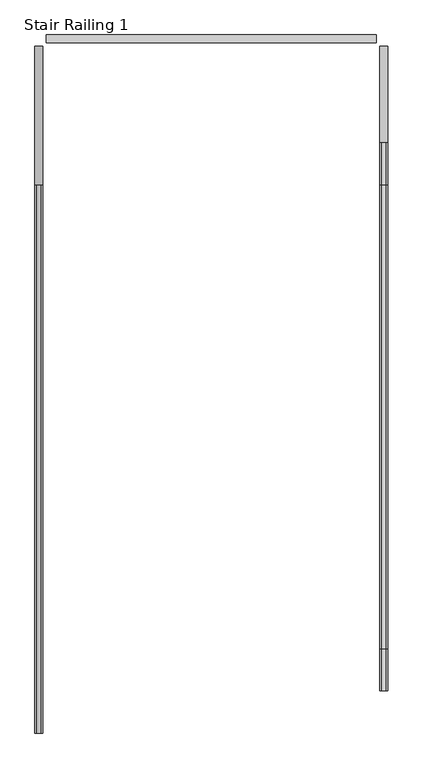
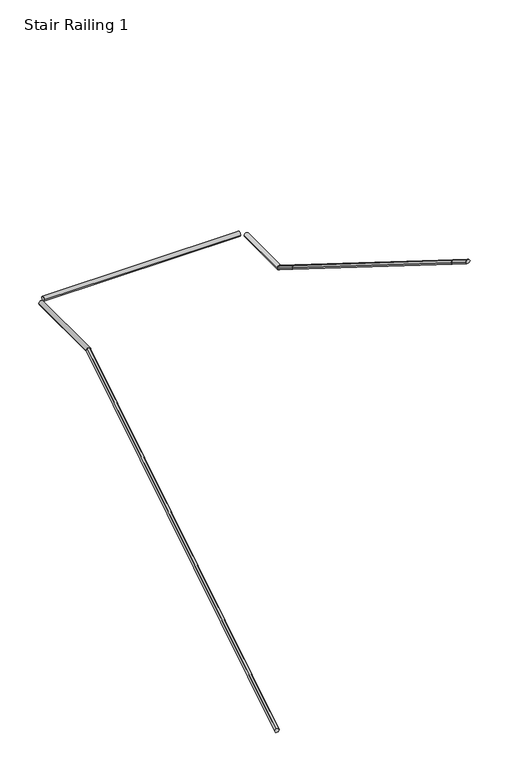
"""IFC4 building model written with IfcOpenShell, lengths in millimetres: railing geometry, Stair Railing 1."""

import ifcopenshell
import ifcopenshell.guid

model = None  # the IFC model being written
_history = None  # IfcOwnerHistory: only IFC2X3 demands one
_inside = {}  # id of a spatial element -> (the spatial element, [elements in it])
_under = {}  # id of a project, library or spatial element -> (it, [spatial elements below it])
_declared = {}  # id of a project -> (the project, [libraries it declares])
_typed = {}  # id of a type object -> (the type object, [elements of that type])
_made_of = {}  # id of a material, layer set ... -> (it, [elements and type objects made of it])


def new_model(schema):
    """Start an empty IFC model of exactly this schema.

    Asked for "IFC4X3", IfcOpenShell would pick the latest addendum, in which some entities
    have other attributes; the version numbers below select the first issue.
    IFC2X3 requires an IfcOwnerHistory on every rooted entity: one is made here for all.
    """
    global model, _history
    if schema == "IFC4X3":
        model = ifcopenshell.file(schema_version=(4, 3, 0, 0))
    else:
        model = ifcopenshell.file(schema=schema)
    _inside.clear()
    _under.clear()
    _declared.clear()
    _typed.clear()
    _made_of.clear()
    _history = None
    if model.schema == "IFC2X3":
        org = make("IfcOrganization", Name="unknown")
        user = make(
            "IfcPersonAndOrganization",
            ThePerson=make("IfcPerson", FamilyName="unknown"),
            TheOrganization=org,
        )
        app = make(
            "IfcApplication",
            ApplicationDeveloper=org,
            Version="unknown",
            ApplicationFullName="unknown",
            ApplicationIdentifier="unknown",
        )
        _history = make(
            "IfcOwnerHistory",
            OwningUser=user,
            OwningApplication=app,
            ChangeAction="ADDED",
            CreationDate=0,
        )
    return model


def make(cls, **values):
    """One entity of the class cls with the attributes given. An attribute that is None is left unset."""
    return model.create_entity(
        cls, **{name: value for name, value in values.items() if value is not None}
    )


def rooted(cls, **values):
    """An entity with a GlobalId (a new one), such as an element, a storey or a relation."""
    return make(cls, GlobalId=ifcopenshell.guid.new(), OwnerHistory=_history, **values)


def si_unit(unit_type, name, prefix=None):
    """IfcSIUnit, for example si_unit("LENGTHUNIT", "METRE", prefix="MILLI")."""
    return make("IfcSIUnit", UnitType=unit_type, Prefix=prefix, Name=name)


def assignment(units):
    """IfcUnitAssignment: the units of a project."""
    return None if units is None else make("IfcUnitAssignment", Units=units)


def point(xyz):
    """IfcCartesianPoint."""
    return None if xyz is None else make("IfcCartesianPoint", Coordinates=xyz)


def direction(xyz):
    """IfcDirection."""
    return None if xyz is None else make("IfcDirection", DirectionRatios=xyz)


def frame(location, z_axis=None, x_axis=None):
    """IfcAxis2Placement3D, a coordinate frame: its origin and axes. An axis left out is left unset."""
    return make(
        "IfcAxis2Placement3D",
        Location=point(location),
        Axis=direction(z_axis),
        RefDirection=direction(x_axis),
    )


def origin():
    """The frame at (0, 0, 0) with its axes left unset."""
    return frame((0.0, 0.0, 0.0))


def place(relative_to, where):
    """IfcLocalPlacement: puts the frame where relative to a parent placement (None: the world)."""
    return make(
        "IfcLocalPlacement", PlacementRelTo=relative_to, RelativePlacement=where
    )


def context(
    kind, dimensions, precision=None, world=None, true_north=None, identifier=None
):
    """IfcGeometricRepresentationContext, for example the 3D "Model" context."""
    return make(
        "IfcGeometricRepresentationContext",
        ContextIdentifier=identifier,
        ContextType=kind,
        CoordinateSpaceDimension=dimensions,
        Precision=precision,
        WorldCoordinateSystem=world,
        TrueNorth=true_north,
    )


def project(units=None, contexts=None):
    """IfcProject with its units and contexts."""
    return rooted(
        "IfcProject",
        Name="project",
        RepresentationContexts=contexts,
        UnitsInContext=assignment(units),
    )


def spatial(cls, under=None, at=None, **own):
    """A site, building, storey or space (cls), placed at a placement, below another one or the project."""
    s = rooted(cls, ObjectPlacement=at, **own)
    if under is not None:
        _under.setdefault(under.id(), (under, []))[1].append(s)
    return s


def circle_curve(where, radius):
    """IfcCircle in the frame where."""
    return make("IfcCircle", Position=where, Radius=radius)


def faces_of(points, faces, orient=None, outer=None):
    """IfcFace entities. A face is a list of loops; a loop is a list of indices into points, from 0.

    orient and outer hold one flag for each loop. By default every Orientation is true, the
    first loop of a face is its IfcFaceOuterBound and the others are IfcFaceBound.
    """
    made = []
    for i, loops in enumerate(faces):
        bounds = []
        for j, loop in enumerate(loops):
            is_outer = j == 0 if outer is None else outer[i][j]
            bounds.append(
                make(
                    "IfcFaceOuterBound" if is_outer else "IfcFaceBound",
                    Bound=make("IfcPolyLoop", Polygon=[points[k] for k in loop]),
                    Orientation=True if orient is None else orient[i][j],
                )
            )
        made.append(make("IfcFace", Bounds=bounds))
    return made


def faceted_brep(points, faces, orient=None, outer=None, voids=None):
    """IfcFacetedBrep: a solid bounded by flat faces; with voids (closed shells), ...WithVoids."""
    shared = [point(p) for p in points]
    hull = make("IfcClosedShell", CfsFaces=faces_of(shared, faces, orient, outer))
    if voids is None:
        return make("IfcFacetedBrep", Outer=hull)
    return make(
        "IfcFacetedBrepWithVoids",
        Outer=hull,
        Voids=[
            make(cls, CfsFaces=faces_of(shared, fs, o, b)) for cls, fs, o, b in voids
        ],
    )


def shape(context_of_items, identifier, shape_type, items):
    """IfcShapeRepresentation: the items that make up one representation, for example the "Body"."""
    return make(
        "IfcShapeRepresentation",
        ContextOfItems=context_of_items,
        RepresentationIdentifier=identifier,
        RepresentationType=shape_type,
        Items=items,
    )


def source(mapping_origin, context_of_items, identifier, shape_type, items):
    """IfcRepresentationMap: a shape defined once, which mapped items show again and again."""
    return make(
        "IfcRepresentationMap",
        MappingOrigin=mapping_origin,
        MappedRepresentation=shape(context_of_items, identifier, shape_type, items),
    )


def transform(
    local_origin,
    x_axis=None,
    y_axis=None,
    z_axis=None,
    scale=None,
    scale2=None,
    scale3=None,
    uniform=True,
):
    """IfcCartesianTransformationOperator3D, or its non-uniform kind. x_axis, y_axis, z_axis: its Axis1, 2, 3."""
    if uniform:
        return make(
            "IfcCartesianTransformationOperator3D",
            Axis1=direction(x_axis),
            Axis2=direction(y_axis),
            LocalOrigin=point(local_origin),
            Scale=scale,
            Axis3=direction(z_axis),
        )
    return make(
        "IfcCartesianTransformationOperator3DnonUniform",
        Axis1=direction(x_axis),
        Axis2=direction(y_axis),
        LocalOrigin=point(local_origin),
        Scale=scale,
        Axis3=direction(z_axis),
        Scale2=scale2,
        Scale3=scale3,
    )


def mapped(mapping_source, mapping_target):
    """IfcMappedItem: shows the shape of a source again, moved by a transform."""
    return make(
        "IfcMappedItem", MappingSource=mapping_source, MappingTarget=mapping_target
    )


def made_of(thing, what):
    """Note that an element or type object is made of a material, layer set ...; save() writes the relation."""
    if what is not None:
        _made_of.setdefault(what.id(), (what, []))[1].append(thing)
    return thing


def element(
    cls,
    number,
    at=None,
    inside=None,
    cuts=None,
    type_object=None,
    material=None,
    context=None,
    identifier="Body",
    shape_type=None,
    held_by="IfcProductDefinitionShape",
    body=None,
    shapes=None,
    **own,
):
    """One element of the class cls, such as IfcWall. Its Tag is "e" and its number.

    at: its placement. inside: the storey or other place that contains it. cuts: it is an
    opening in that element (IfcRelVoidsElement). A single representation is given by context,
    identifier, shape_type and body (its items); several are given by shapes. held_by: the class
    of the entity that holds the representations. save() writes the other relations.
    """
    e = rooted(cls, Tag="e%d" % number, ObjectPlacement=at, **own)
    if body is not None:
        shapes = [shape(context, identifier, shape_type, body)]
    if shapes is not None:
        e.Representation = make(held_by, Representations=shapes)
    if inside is not None:
        _inside.setdefault(inside.id(), (inside, []))[1].append(e)
    if cuts is not None:
        rooted(
            "IfcRelVoidsElement", RelatingBuildingElement=cuts, RelatedOpeningElement=e
        )
    if type_object is not None:
        _typed.setdefault(type_object.id(), (type_object, []))[1].append(e)
    return made_of(e, material)


def aggregate(whole, parts):
    """IfcRelAggregates: a whole, such as a stair, and the parts it consists of."""
    return rooted("IfcRelAggregates", RelatingObject=whole, RelatedObjects=parts)


def save(model, path):
    """Write the relations noted so far, then the file.

    IfcRelAggregates (storeys below a building ...), IfcRelContainedInSpatialStructure (elements
    in a storey), IfcRelDefinesByType, IfcRelAssociatesMaterial and IfcRelDeclares: one each for
    every whole, place, type object, material and project.
    """
    for whole, parts in _under.values():
        aggregate(whole, parts)
    for where, things in _inside.values():
        rooted(
            "IfcRelContainedInSpatialStructure",
            RelatedElements=things,
            RelatingStructure=where,
        )
    for kind, things in _typed.values():
        rooted("IfcRelDefinesByType", RelatedObjects=things, RelatingType=kind)
    for what, things in _made_of.values():
        rooted("IfcRelAssociatesMaterial", RelatedObjects=things, RelatingMaterial=what)
    for by, libraries in _declared.values():
        rooted("IfcRelDeclares", RelatingContext=by, RelatedDefinitions=libraries)
    model.write(path)


def plane_surface(at):
    """IfcPlane: the flat surface through the origin of the frame at, square to its z axis."""
    return make("IfcPlane", Position=at)


def cylinder_surface(at, radius):
    """IfcCylindricalSurface: all points at the distance radius from the z axis of the frame at."""
    return make("IfcCylindricalSurface", Position=at, Radius=radius)


def advanced_brep(points, edges, surfaces, faces):
    """IfcAdvancedBrep: a solid bounded by faces that lie on surfaces and meet in shared edges.

    An edge is (start, end): straight between two places in points (the first is 0);
    or (start, end, curve); or (start, end, curve, False) where it runs against its curve.
    A face is (place in surfaces, loops), or (place, loops, False) where it looks against
    its surface's normal. A loop lists edges by number (the first is 1), with a minus sign
    where the edge is run from its end to its start. The first loop is the outer one.
    """
    corners = [point(p) for p in points]
    vertices = [make("IfcVertexPoint", VertexGeometry=c) for c in corners]
    made = []
    for start, end, *more in edges:
        made.append(
            make(
                "IfcEdgeCurve",
                EdgeStart=vertices[start],
                EdgeEnd=vertices[end],
                EdgeGeometry=more[0] if more else make("IfcPolyline", Points=[corners[start], corners[end]]),
                SameSense=more[1] if len(more) > 1 else True,
            )
        )
    hull = []
    for where, loops, *sense in faces:
        bounds = []
        for j, loop in enumerate(loops):
            ring = [make("IfcOrientedEdge", EdgeElement=made[abs(k) - 1], Orientation=k > 0) for k in loop]
            bounds.append(
                make(
                    "IfcFaceOuterBound" if j == 0 else "IfcFaceBound",
                    Bound=make("IfcEdgeLoop", EdgeList=ring),
                    Orientation=True,
                )
            )
        hull.append(make("IfcAdvancedFace", Bounds=bounds, FaceSurface=surfaces[where], SameSense=sense[0] if sense else True))
    return make("IfcAdvancedBrep", Outer=make("IfcClosedShell", CfsFaces=hull))


def stair_railing_1_2cf15c4a(model_context):
    return source(origin(), model_context, "Body", "SolidModel", [
        faceted_brep([(-2482.1134126, 56357.2066802, 13752.6888889), (-2469.4134126, 56357.2066802, 13774.6859341), (-2444.0134126, 56357.2066802, 13774.6859341), (-2431.3134126, 56357.2066802, 13752.6888889), (-2444.0134126, 56357.2066802, 13730.6918436), (-2469.4134126, 56357.2066802, 13730.6918436), (-2482.1134126, 52725.0066802, 11477.9777778), (-2469.4134126, 52725.0066802, 11455.9807325), (-2444.0134126, 52725.0066802, 11455.9807325), (-2431.3134126, 52725.0066802, 11477.9777778), (-2444.0134126, 52725.0066802, 11499.974823), (-2469.4134126, 52725.0066802, 11499.974823)], [[[0, 1, 2, 3, 4, 5]], [[6, 7, 8, 9, 10, 11]], [[1, 0, 6, 11]], [[2, 1, 11, 10]], [[3, 2, 10, 9]], [[4, 3, 9, 8]], [[5, 4, 8, 7]], [[0, 5, 7, 6]]]),
        advanced_brep(
        [(-2482.1134126, 57271.6066802, 13752.6888889), (-2431.3134126, 57271.6066802, 13752.6888889), (-2482.1134126, 56357.2066802, 13752.6888889), (-2431.3134126, 56357.2066802, 13752.6888889)],
        [
            (0, 1, circle_curve(frame((-2456.7134126, 57271.6066802, 13752.6888889), z_axis=(0.0, 1.0, 0.0), x_axis=(-0.9999999999999999, 0.0, 0.0)), 25.4)),
            (1, 0, circle_curve(frame((-2456.7134126, 57271.6066802, 13752.6888889), z_axis=(0.0, 1.0, 0.0), x_axis=(-0.9999999999999999, 0.0, 0.0)), 25.4)),
            (2, 3, circle_curve(frame((-2456.7134126, 56357.2066802, 13752.6888889), z_axis=(0.0, -1.0, 0.0), x_axis=(-0.9999999999999999, 0.0, 0.0)), 25.4)),
            (3, 2, circle_curve(frame((-2456.7134126, 56357.2066802, 13752.6888889), z_axis=(0.0, -1.0, 0.0), x_axis=(-0.9999999999999999, 0.0, 0.0)), 25.4)),
            (0, 2),
            (3, 1),
        ],
        [
            plane_surface(frame((-2482.1134126, 57271.6066802, 13727.2888889), z_axis=(0.0, 1.0, 0.0), x_axis=(0.0, 0.0, 1.0))),
            plane_surface(frame((-2482.1134126, 56357.2066802, 13727.2888889), z_axis=(0.0, -1.0, 0.0), x_axis=(0.0, 0.0, -1.0))),
            cylinder_surface(frame((-2456.7134126, 56357.2066802, 13752.6888889), z_axis=(0.0, 0.9999999999999999, 0.0), x_axis=(-0.9999999999999999, 0.0, 0.0)), 25.4),
        ],
        [
            (0, [[1, 2]]),
            (1, [[3, 4]]),
            (2, [[-1, 5, -4, 6]]),
            (2, [[-2, -6, -3, -5]]),
        ],
    ),
        advanced_brep(
        [(-222.5891104, 57347.8066802, 13752.6888889), (-222.5891104, 57297.0066802, 13752.6888889), (-2405.9134126, 57347.8066802, 13752.6888889), (-2405.9134126, 57297.0066802, 13752.6888889)],
        [
            (0, 1, circle_curve(frame((-222.5891104, 57322.4066802, 13752.6888889), z_axis=(1.0, 0.0, 0.0), x_axis=(0.0, 1.0, 0.0)), 25.4)),
            (1, 0, circle_curve(frame((-222.5891104, 57322.4066802, 13752.6888889), z_axis=(1.0, 0.0, 0.0), x_axis=(0.0, 1.0, 0.0)), 25.4)),
            (2, 3, circle_curve(frame((-2405.9134126, 57322.4066802, 13752.6888889), z_axis=(-1.0, 0.0, 0.0), x_axis=(0.0, 1.0, 0.0)), 25.4)),
            (3, 2, circle_curve(frame((-2405.9134126, 57322.4066802, 13752.6888889), z_axis=(-1.0, 0.0, 0.0), x_axis=(0.0, 1.0, 0.0)), 25.4)),
            (0, 2),
            (3, 1),
        ],
        [
            plane_surface(frame((-222.5891104, 57347.8066802, 13727.2888889), z_axis=(1.0, 0.0, 0.0), x_axis=(0.0, 1.0, 0.0))),
            plane_surface(frame((-2405.9134126, 57347.8066802, 13727.2888889), z_axis=(-1.0, 0.0, 0.0), x_axis=(0.0, -1.0, 0.0))),
            cylinder_surface(frame((-2405.9134126, 57322.4066802, 13752.6888889), z_axis=(1.0, 0.0, 0.0), x_axis=(0.0, 1.0, 0.0)), 25.4),
        ],
        [
            (0, [[1, 2]]),
            (1, [[3, 4]]),
            (2, [[-1, 5, -4, 6]]),
            (2, [[-2, -6, -3, -5]]),
        ],
    ),
        advanced_brep(
        [(-146.3891104, 56636.6066802, 13752.6888889), (-197.1891104, 56636.6066802, 13752.6888889), (-146.3891104, 57271.6066802, 13752.6888889), (-197.1891104, 57271.6066802, 13752.6888889)],
        [
            (0, 1, circle_curve(frame((-171.7891104, 56636.6066802, 13752.6888889), z_axis=(0.0, -1.0, 0.0), x_axis=(1.0, 0.0, 0.0)), 25.4)),
            (1, 0, circle_curve(frame((-171.7891104, 56636.6066802, 13752.6888889), z_axis=(0.0, -1.0, 0.0), x_axis=(1.0, 0.0, 0.0)), 25.4)),
            (2, 3, circle_curve(frame((-171.7891104, 57271.6066802, 13752.6888889), z_axis=(0.0, 1.0, 0.0), x_axis=(1.0, 0.0, 0.0)), 25.4)),
            (3, 2, circle_curve(frame((-171.7891104, 57271.6066802, 13752.6888889), z_axis=(0.0, 1.0, 0.0), x_axis=(1.0, 0.0, 0.0)), 25.4)),
            (0, 2),
            (3, 1),
        ],
        [
            plane_surface(frame((-146.3891104, 56636.6066802, 13727.2888889), z_axis=(0.0, -1.0, 0.0), x_axis=(0.0, 0.0, -1.0))),
            plane_surface(frame((-146.3891104, 57271.6066802, 13727.2888889), z_axis=(0.0, 1.0, 0.0), x_axis=(0.0, 0.0, 1.0))),
            cylinder_surface(frame((-171.7891104, 57271.6066802, 13752.6888889), z_axis=(0.0, -1.0, 0.0), x_axis=(1.0, 0.0, 0.0)), 25.4),
        ],
        [
            (0, [[1, 2]]),
            (1, [[3, 4]]),
            (2, [[-1, 5, -4, 6]]),
            (2, [[-2, -6, -3, -5]]),
        ],
    ),
        faceted_brep([(-146.3891104, 56357.2066802, 13927.6666667), (-159.0891104, 56357.2066802, 13949.6637119), (-184.4891104, 56357.2066802, 13949.6637119), (-197.1891104, 56357.2066802, 13927.6666667), (-184.4891104, 56357.2066802, 13905.6696214), (-159.0891104, 56357.2066802, 13905.6696214), (-146.3891104, 56636.6066802, 13752.6888889), (-159.0891104, 56636.6066802, 13730.6918436), (-184.4891104, 56636.6066802, 13730.6918436), (-197.1891104, 56636.6066802, 13752.6888889), (-184.4891104, 56636.6066802, 13774.6859341), (-159.0891104, 56636.6066802, 13774.6859341)], [[[0, 1, 2, 3, 4, 5]], [[6, 7, 8, 9, 10, 11]], [[1, 0, 6, 11]], [[2, 1, 11, 10]], [[3, 2, 10, 9]], [[4, 3, 9, 8]], [[5, 4, 8, 7]], [[0, 5, 7, 6]]]),
        faceted_brep([(-146.3891104, 53283.8066802, 15852.4222222), (-159.0891104, 53283.8066802, 15874.4192675), (-184.4891104, 53283.8066802, 15874.4192675), (-197.1891104, 53283.8066802, 15852.4222222), (-184.4891104, 53283.8066802, 15830.425177), (-159.0891104, 53283.8066802, 15830.425177), (-146.3891104, 56357.2066802, 13927.6666667), (-159.0891104, 56357.2066802, 13905.6696214), (-184.4891104, 56357.2066802, 13905.6696214), (-197.1891104, 56357.2066802, 13927.6666667), (-184.4891104, 56357.2066802, 13949.6637119), (-159.0891104, 56357.2066802, 13949.6637119)], [[[0, 1, 2, 3, 4, 5]], [[6, 7, 8, 9, 10, 11]], [[1, 0, 6, 11]], [[2, 1, 11, 10]], [[3, 2, 10, 9]], [[4, 3, 9, 8]], [[5, 4, 8, 7]], [[0, 5, 7, 6]]]),
        faceted_brep([(-146.3891104, 53004.4066802, 16027.4), (-159.0891104, 53004.4066802, 16049.3970453), (-184.4891104, 53004.4066802, 16049.3970453), (-197.1891104, 53004.4066802, 16027.4), (-184.4891104, 53004.4066802, 16005.4029547), (-159.0891104, 53004.4066802, 16005.4029547), (-146.3891104, 53283.8066802, 15852.4222222), (-159.0891104, 53283.8066802, 15830.425177), (-184.4891104, 53283.8066802, 15830.425177), (-197.1891104, 53283.8066802, 15852.4222222), (-184.4891104, 53283.8066802, 15874.4192675), (-159.0891104, 53283.8066802, 15874.4192675)], [[[0, 1, 2, 3, 4, 5]], [[6, 7, 8, 9, 10, 11]], [[1, 0, 6, 11]], [[2, 1, 11, 10]], [[3, 2, 10, 9]], [[4, 3, 9, 8]], [[5, 4, 8, 7]], [[0, 5, 7, 6]]]),
    ])


if __name__ == "__main__":
    model = new_model("IFC4")
    model_context = context("Model", 3, world=origin())
    ifc_project = project(units=[si_unit("LENGTHUNIT", "METRE", prefix="MILLI")], contexts=[model_context])
    site = spatial("IfcSite", under=ifc_project)
    building = spatial("IfcBuilding", under=site)
    placement = place(None, origin())
    stair_railing_1_shape = stair_railing_1_2cf15c4a(model_context)
    element("IfcRailing", 1, ObjectType="Stair Railing 1", at=placement, inside=building, context=model_context, shape_type="MappedRepresentation", body=[
        mapped(stair_railing_1_shape, transform((0.0, 0.0, 0.0), x_axis=(1.0, 0.0, 0.0), y_axis=(0.0, 1.0, 0.0), z_axis=(0.0, 0.0, 1.0))),
    ])
    save(model, "model.ifc")
